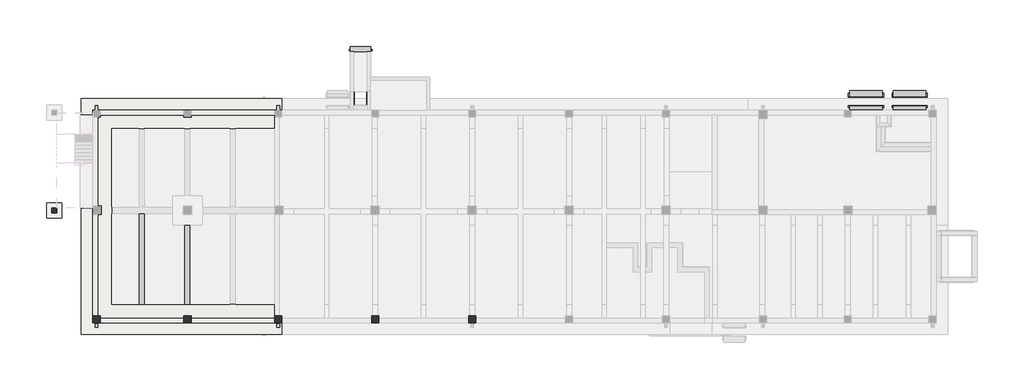
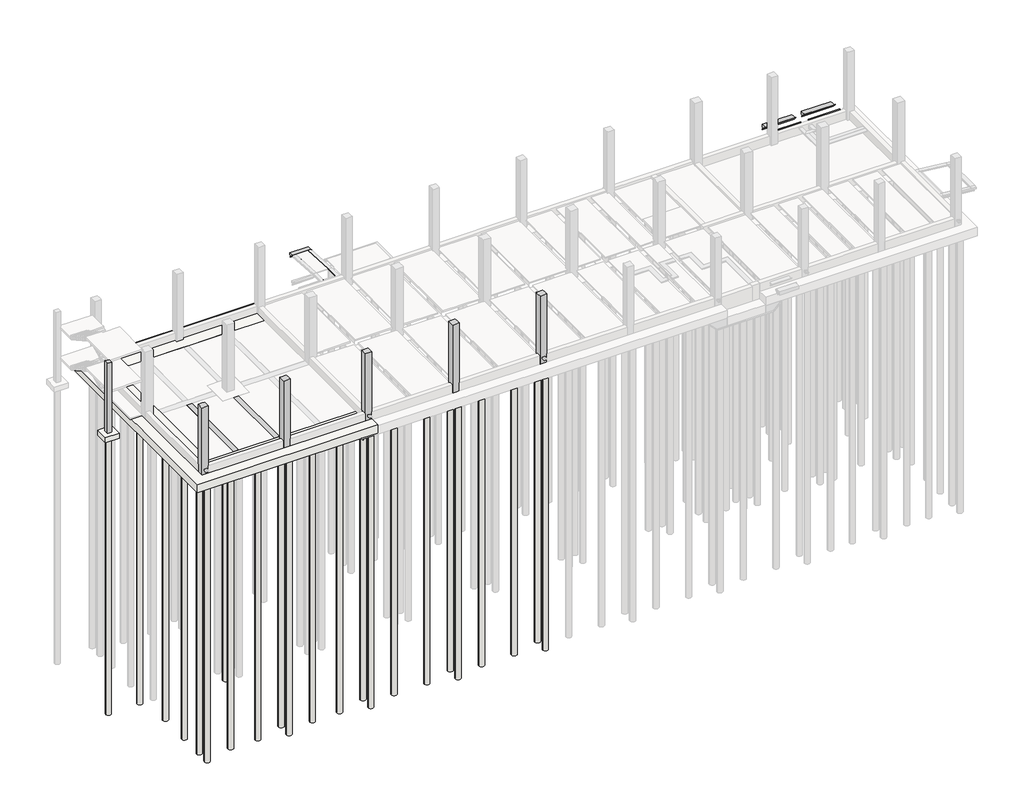
# One storey, part 3 of 7: 26 slabs, 11 proxies, 6 columns, 2 beams.
"""IFC4 building model written with IfcOpenShell, lengths in millimetres."""

from ifc_helpers import new_model, si_unit, point, frame, frame_2d, origin, place, context, project, spatial, polyline, circle_curve, trimmed, segment, composite_curve, outline, extrude, faceted_brep, element, save

model = new_model("IFC4")

# Units and contexts
model_context = context("Model", 3, world=origin())
ifc_project = project(units=[si_unit("LENGTHUNIT", "METRE", prefix="MILLI")], contexts=[model_context])

# Site, building, storey
site = spatial("IfcSite", under=ifc_project)
building = spatial("IfcBuilding", under=site)
storey = spatial("IfcBuildingStorey", under=building, Name="H.P.P", Elevation=4500.0)

# Beams
placement = place(None, origin())
element("IfcBeam", 1, ObjectType="RC Beam_Rectangular : H_SB_AR S16_TG-UG_500x700_FB1A", at=placement, inside=storey, context=model_context, shape_type="Brep", body=[
    faceted_brep([(3500.0, -15750.0, 3400.0), (4000.0, -15750.0, 3400.0), (4000.0, -15750.0, 3840.0), (4000.0, -15750.0, 3950.0), (4000.0, -15750.0, 4100.0), (3500.0, -15750.0, 4100.0), (3500.0, -15750.0, 3950.0), (3500.0, -15750.0, 3840.0), (4000.0, -8300.0, 4100.0), (3500.0, -8300.0, 4100.0), (4000.0, -8300.0, 3950.0), (4000.0, -8300.0, 3400.0), (4000.0, -8300.0, 3840.0), (3500.0, -8300.0, 3400.0), (3500.0, -8300.0, 3950.0), (3500.0, -8300.0, 3840.0)], [[[0, 1, 2, 3, 4, 5, 6, 7]], [[5, 4, 8, 9]], [[10, 8, 4, 3, 2, 1, 11, 12]], [[1, 0, 13, 11]], [[9, 14, 15, 13, 0, 7, 6, 5]], [[9, 8, 10, 12, 11, 13, 15, 14]]]),
])
element("IfcBeam", 2, ObjectType="RC Beam_Rectangular : H_SB_AR S16_TG-UG_500x700_FG1", at=placement, inside=storey, context=model_context, shape_type="Brep", body=[
    faceted_brep([(7250.0, -9250.0, 4100.0), (7750.0, -9250.0, 4100.0), (7750.0, -9250.0, 3950.0), (7750.0, -9250.0, 3840.0), (7750.0, -9250.0, 3400.0), (7250.0, -9250.0, 3400.0), (7250.0, -9250.0, 3840.0), (7250.0, -9250.0, 3950.0), (7250.0, -15750.0, 3400.0), (7750.0, -15750.0, 3400.0), (7750.0, -15750.0, 3840.0), (7750.0, -15750.0, 3950.0), (7750.0, -15750.0, 4100.0), (7250.0, -15750.0, 4100.0), (7250.0, -15750.0, 3950.0), (7250.0, -15750.0, 3840.0)], [[[0, 1, 2, 3, 4, 5, 6, 7]], [[8, 9, 10, 11, 12, 13, 14, 15]], [[1, 0, 13, 12]], [[1, 12, 11, 10, 9, 4, 3, 2]], [[5, 4, 9, 8]], [[13, 0, 7, 6, 5, 8, 15, 14]]]),
])

# Proxies
element("IfcBuildingElementProxy", 3, Name="H_SF_AR_B08_Stoop_T150_FrontEdge", ObjectType="H_SF_AR_B08_Stoop_T150_FrontEdge", at=placement, inside=storey, context=model_context, shape_type="SweptSolid", body=[
    extrude(outline(polyline([(312.0000074, 4450.0), (312.0000074, 4600.0), (662.0000074, 4600.0), (512.0000074, 4450.0), (312.0000074, 4450.0)])), frame((65750.0, 0.0, 0.0), z_axis=(1.0, 0.0, 0.0), x_axis=(0.0, 1.0, 0.0)), (0.0, 0.0, 1.0), 2700.0),
])
element("IfcBuildingElementProxy", 4, Name="H_SF_AR_B08_Stoop_T150_FrontEdge_500x300", ObjectType="H_SF_AR_B08_Stoop_T150_FrontEdge_500x300", at=placement, inside=storey, context=model_context, shape_type="Brep", body=[
    faceted_brep([(68450.0, 1900.0, 4300.0), (68450.0, 1900.0, 4600.0), (68450.0, 1600.0, 4600.0), (68450.0, 1400.0, 4600.0), (68450.0, 1700.0, 4300.0), (65750.0, 1900.0, 4300.0), (65750.0, 1700.0, 4300.0), (65750.0, 1400.0, 4600.0), (65750.0, 1600.0, 4600.0), (65750.0, 1900.0, 4600.0)], [[[0, 1, 2, 3, 4]], [[5, 6, 7, 8, 9]], [[1, 0, 5, 9]], [[3, 2, 1, 9, 8, 7]], [[4, 3, 7, 6]], [[0, 4, 6, 5]]]),
])
element("IfcBuildingElementProxy", 5, Name="H_SF_AR_S18_Lean_T50_300X300", ObjectType="H_SF_AR_S18_Lean_T50_300X300", at=placement, inside=storey, context=model_context, shape_type="SweptSolid", body=[
    extrude(outline(polyline([(1700.0, 4300.0), (1700.0, 4250.0), (1679.2893219, 4250.0), (1379.2893219, 4550.0), (1400.0, 4550.0), (1400.0, 4600.0), (1700.0, 4300.0)])), frame((65650.0, 0.0, 0.0), z_axis=(1.0, 0.0, 0.0), x_axis=(0.0, 1.0, 0.0)), (0.0, 0.0, 1.0), 2900.0),
])
element("IfcBuildingElementProxy", 6, Name="H_SF_AR_S18_Lean_T50_150X150", ObjectType="H_SF_AR_S18_Lean_T50_150X150", at=placement, inside=storey, context=model_context, shape_type="SweptSolid", body=[
    extrude(outline(polyline([(512.0000074, 4400.0), (512.0000074, 4450.0), (662.0000074, 4600.0), (662.0000074, 4550.0), (682.7106855, 4550.0), (532.7106855, 4400.0), (512.0000074, 4400.0)])), frame((65650.0, 0.0, 0.0), z_axis=(1.0, 0.0, 0.0), x_axis=(0.0, 1.0, 0.0)), (0.0, 0.0, 1.0), 2900.0),
])
element("IfcBuildingElementProxy", 7, Name="H_SF_AR_B08_Stoop_T150_FrontEdge", ObjectType="H_SF_AR_B08_Stoop_T150_FrontEdge", at=placement, inside=storey, context=model_context, shape_type="SweptSolid", body=[
    extrude(outline(polyline([(312.0000074, 4450.0), (312.0000074, 4600.0), (662.0000074, 4600.0), (512.0000074, 4450.0), (312.0000074, 4450.0)])), frame((62150.0, 0.0, 0.0), z_axis=(1.0, 0.0, 0.0), x_axis=(0.0, 1.0, 0.0)), (0.0, 0.0, 1.0), 2700.0),
])
element("IfcBuildingElementProxy", 8, Name="H_SF_AR_B08_Stoop_T150_FrontEdge_500x300", ObjectType="H_SF_AR_B08_Stoop_T150_FrontEdge_500x300", at=placement, inside=storey, context=model_context, shape_type="Brep", body=[
    faceted_brep([(64850.0, 1900.0, 4300.0), (64850.0, 1900.0, 4600.0), (64850.0, 1600.0, 4600.0), (64850.0, 1400.0, 4600.0), (64850.0, 1700.0, 4300.0), (62150.0, 1900.0, 4300.0), (62150.0, 1700.0, 4300.0), (62150.0, 1400.0, 4600.0), (62150.0, 1600.0, 4600.0), (62150.0, 1900.0, 4600.0)], [[[0, 1, 2, 3, 4]], [[5, 6, 7, 8, 9]], [[1, 0, 5, 9]], [[3, 2, 1, 9, 8, 7]], [[4, 3, 7, 6]], [[0, 4, 6, 5]]]),
])
element("IfcBuildingElementProxy", 9, Name="H_SF_AR_S18_Lean_T50_300X300", ObjectType="H_SF_AR_S18_Lean_T50_300X300", at=placement, inside=storey, context=model_context, shape_type="SweptSolid", body=[
    extrude(outline(polyline([(1700.0, 4300.0), (1700.0, 4250.0), (1679.2893219, 4250.0), (1379.2893219, 4550.0), (1400.0, 4550.0), (1400.0, 4600.0), (1700.0, 4300.0)])), frame((62050.0, 0.0, 0.0), z_axis=(1.0, 0.0, 0.0), x_axis=(0.0, 1.0, 0.0)), (0.0, 0.0, 1.0), 2900.0),
])
element("IfcBuildingElementProxy", 10, Name="H_SF_AR_S18_Lean_T50_150X150", ObjectType="H_SF_AR_S18_Lean_T50_150X150", at=placement, inside=storey, context=model_context, shape_type="SweptSolid", body=[
    extrude(outline(polyline([(512.0000074, 4400.0), (512.0000074, 4450.0), (662.0000074, 4600.0), (662.0000074, 4550.0), (682.7106855, 4550.0), (532.7106855, 4400.0), (512.0000074, 4400.0)])), frame((62050.0, 0.0, 0.0), z_axis=(1.0, 0.0, 0.0), x_axis=(0.0, 1.0, 0.0)), (0.0, 0.0, 1.0), 2900.0),
])
element("IfcBuildingElementProxy", 11, Name="H_SF_AR_B08_Ramp_T150_FrontEdge(SLOPE)", ObjectType="H_SF_AR_B08_Ramp_T150_FrontEdge(SLOPE)", at=placement, inside=storey, context=model_context, shape_type="Brep", body=[
    faceted_brep([(22638.0, 5300.0, 4179.6670362), (22638.0, 5550.0, 4179.6670362), (22638.0, 5550.0, 4349.6670362), (22638.0, 5100.0, 4379.6670362), (22638.0, 5261.0710326, 4218.5960036), (20938.0, 5550.0, 4179.6670362), (20938.0, 5300.0, 4179.6670362), (20938.0, 5261.0710326, 4218.5960036), (20938.0, 5100.0, 4379.6670362), (20938.0, 5550.0, 4349.6670362), (22338.0, 5100.0, 4379.6670362), (21238.0, 5100.0, 4379.6670362)], [[[0, 1, 2, 3, 4]], [[5, 6, 7, 8, 9]], [[1, 5, 9, 2]], [[1, 0, 6, 5]], [[0, 4, 3, 10, 11, 8, 7, 6]], [[3, 2, 9, 8, 11, 10]]]),
])
element("IfcBuildingElementProxy", 12, Name="H_SF_AR_S18_Lean_T50_200X200", ObjectType="H_SF_AR_S18_Lean_T50_200X200", at=placement, inside=storey, context=model_context, shape_type="Brep", body=[
    faceted_brep([(20838.0, 5300.0, 4179.6670362), (20838.0, 5300.0, 4129.6670362), (20838.0, 5279.2893219, 4129.6670362), (20838.0, 5184.596098, 4224.3602601), (20838.0, 5260.3575388, 4219.3094974), (22738.0, 5300.0, 4129.6670362), (22738.0, 5300.0, 4179.6670362), (22738.0, 5260.3575388, 4219.3094974), (22738.0, 5184.596098, 4224.3602601), (22738.0, 5238.2864422, 4170.6699159), (22738.0, 5279.2893219, 4129.6670362), (20938.0, 5260.3575388, 4219.3094974), (20938.0, 5261.0710326, 4218.5960036), (21088.0, 5261.0710326, 4218.5960036), (21238.0, 5100.0, 4379.6670362), (22338.0, 5100.0, 4379.6670362), (22488.0, 5261.0710326, 4218.5960036), (22638.0, 5261.0710326, 4218.5960036), (22638.0, 5260.3575388, 4219.3094974), (22638.0, 5300.0, 4179.6670362), (20938.0, 5300.0, 4179.6670362), (22638.0, 5184.596098, 4224.3602601), (22638.0, 5185.3095918, 4223.6467663), (22488.0, 5185.3095918, 4223.6467663), (22389.2669117, 5079.2893219, 4329.6670362), (22319.2206862, 5079.2893219, 4329.6670362), (21256.7793138, 5079.2893219, 4329.6670362), (21186.7330883, 5079.2893219, 4329.6670362), (21088.0, 5185.3095918, 4223.6467663), (20938.0, 5185.3095918, 4223.6467663), (20938.0, 5184.596098, 4224.3602601), (20850.0, 5184.596098, 4224.3602601), (22387.8892579, 5100.0, 4329.6670362), (22317.8430324, 5100.0, 4329.6670362), (21258.1569676, 5100.0, 4329.6670362), (21188.1107421, 5100.0, 4329.6670362)], [[[0, 1, 2, 3, 4]], [[5, 6, 7, 8, 9, 10]], [[0, 4, 11, 12, 13, 14, 15, 16, 17, 18, 7, 6, 19, 20]], [[1, 0, 20, 19, 6, 5]], [[2, 1, 5, 10]], [[2, 10, 9, 8, 21, 22, 23, 24, 25, 26, 27, 28, 29, 30, 31, 3]], [[27, 26, 25, 24, 32, 33, 34, 35]], [[15, 14, 35, 34, 33, 32]], [[8, 7, 18, 21]], [[4, 3, 31, 30, 11]], [[29, 12, 11, 30]], [[13, 28, 27, 35, 14]], [[12, 29, 28, 13]], [[17, 22, 21, 18]], [[23, 16, 15, 32, 24]], [[22, 17, 16, 23]]]),
])
element("IfcBuildingElementProxy", 13, Name="H_SF_AR_S18_Lean_T50_150X150", ObjectType="H_SF_AR_S18_Lean_T50_150X150", at=placement, inside=storey, context=model_context, shape_type="Brep", body=[
    faceted_brep([(22338.0, 1800.0, 4600.0), (22488.0, 1800.0, 4450.0), (22488.0, 1800.0, 4400.0), (22467.2893219, 1800.0, 4400.0), (22317.2893219, 1800.0, 4550.0), (22338.0, 1800.0, 4550.0), (22488.0, 550.0, 4450.0), (22338.0, 700.0, 4600.0), (22338.0, 700.0, 4550.0), (22317.2893219, 720.7106781, 4550.0), (22467.2893219, 570.7106781, 4400.0), (22488.0, 550.0, 4400.0)], [[[0, 1, 2, 3, 4, 5]], [[6, 7, 8, 9, 10, 11]], [[1, 0, 7, 6]], [[2, 1, 6, 11]], [[3, 2, 11, 10]], [[4, 3, 10, 9]], [[5, 4, 9, 8]], [[0, 5, 8, 7]]]),
    faceted_brep([(21238.0, 700.0, 4600.0), (21088.0, 550.0, 4450.0), (21088.0, 550.0, 4400.0), (21108.7106781, 570.7106781, 4400.0), (21258.7106781, 720.7106781, 4550.0), (21238.0, 700.0, 4550.0), (21088.0, 1800.0, 4450.0), (21238.0, 1800.0, 4600.0), (21238.0, 1800.0, 4550.0), (21258.7106781, 1800.0, 4550.0), (21108.7106781, 1800.0, 4400.0), (21088.0, 1800.0, 4400.0)], [[[0, 1, 2, 3, 4, 5]], [[6, 7, 8, 9, 10, 11]], [[1, 0, 7, 6]], [[2, 1, 6, 11]], [[3, 2, 11, 10]], [[4, 3, 10, 9]], [[5, 4, 9, 8]], [[0, 5, 8, 7]]]),
    faceted_brep([(22488.0, 1800.0, 4450.0), (22338.0, 1800.0, 4600.3329638), (22338.0, 1800.0, 4550.2219759), (22317.2893219, 1800.0, 4550.2219759), (22467.2893219, 1800.0, 4399.8890121), (22488.0, 1800.0, 4399.8890121), (22488.0, 5184.596098, 4224.3602601), (22389.9313644, 5079.2893219, 4329.6670362), (22388.5537105, 5100.0, 4329.6670362), (22338.6644526, 5100.0, 4379.6670362), (22338.0, 5109.9889135, 4379.6670362), (22488.0, 5238.2864422, 4170.6699159), (22467.2893219, 5238.2864422, 4170.6699159), (22317.2893219, 5100.0, 4330.2219759), (22317.8430324, 5100.0, 4329.6670362), (22319.2206862, 5079.2893219, 4329.6670362), (22338.0, 5100.0, 4330.2219759), (22338.0, 5100.0, 4379.6670362), (22389.2669117, 5079.2893219, 4329.6670362), (22387.8892579, 5100.0, 4329.6670362)], [[[0, 1, 2, 3, 4, 5]], [[1, 0, 6, 7, 8, 9, 10]], [[0, 5, 11, 6]], [[5, 4, 12, 11]], [[4, 3, 13, 14, 15, 12]], [[3, 2, 16, 13]], [[2, 1, 10, 17, 16]], [[10, 9, 17]], [[15, 18, 7, 6, 11, 12]], [[7, 18, 15, 14, 19, 8]], [[8, 19, 14, 13, 16, 17, 9]]]),
    faceted_brep([(21238.0, 1800.0, 4600.3329638), (21088.0, 1800.0, 4450.0), (21088.0, 1800.0, 4399.8890121), (21108.7106781, 1800.0, 4399.8890121), (21258.7106781, 1800.0, 4550.2219759), (21238.0, 1800.0, 4550.2219759), (21238.0, 5109.9889135, 4379.6670362), (21237.3355474, 5100.0, 4379.6670362), (21187.4462895, 5100.0, 4329.6670362), (21186.0686356, 5079.2893219, 4329.6670362), (21088.0, 5184.596098, 4224.3602601), (21088.0, 5238.2864422, 4170.6699159), (21108.7106781, 5238.2864422, 4170.6699159), (21256.7793138, 5079.2893219, 4329.6670362), (21258.1569676, 5100.0, 4329.6670362), (21258.7106781, 5100.0, 4330.2219759), (21238.0, 5100.0, 4330.2219759), (21238.0, 5100.0, 4379.6670362), (21186.7330883, 5079.2893219, 4329.6670362), (21188.1107421, 5100.0, 4329.6670362)], [[[0, 1, 2, 3, 4, 5]], [[1, 0, 6, 7, 8, 9, 10]], [[2, 1, 10, 11]], [[3, 2, 11, 12]], [[4, 3, 12, 13, 14, 15]], [[5, 4, 15, 16]], [[0, 5, 16, 17, 6]], [[7, 6, 17]], [[9, 18, 13, 12, 11, 10]], [[13, 18, 9, 8, 19, 14]], [[14, 19, 8, 7, 17, 16, 15]]]),
])

# Columns
element("IfcColumn", 14, ObjectType="RC_Column_Rectangular : H_SC_AR S15_RC Col-AG_600x600_C2", at=placement, inside=storey, context=model_context, shape_type="Brep", body=[
    faceted_brep([(30700.0, -16700.0, 4000.0), (31300.0, -16700.0, 4000.0), (31300.0, -16900.0, 4000.0), (31300.0, -17300.0, 4000.0), (30700.0, -17300.0, 4000.0), (30700.0, -16900.0, 4000.0), (30700.0, -16700.0, 4650.0), (30700.0, -16700.0, 4800.0), (30700.0, -16700.0, 10450.0), (30700.0, -16700.0, 10600.0), (30750.0000002, -16700.0, 10600.0), (31249.9999998, -16700.0, 10600.0), (31300.0, -16700.0, 10600.0), (31300.0, -16700.0, 10450.0), (31300.0, -16700.0, 4800.0), (31300.0, -16700.0, 4650.0), (31300.0, -16900.0, 10600.0), (31300.0, -17300.0, 10600.0), (31300.0, -17300.0, 9800.0), (31300.0, -17300.0, 4800.0), (30700.0, -17300.0, 10600.0), (30700.0, -17300.0, 9800.0), (30700.0, -17300.0, 4800.0), (30700.0, -16900.0, 10600.0)], [[[0, 1, 2, 3, 4, 5]], [[1, 0, 6, 7, 8, 9, 10, 11, 12, 13, 14, 15]], [[3, 2, 1, 15, 14, 13, 12, 16, 17, 18, 19]], [[4, 3, 19, 18, 17, 20, 21, 22]], [[0, 5, 4, 22, 21, 20, 23, 9, 8, 7, 6]], [[20, 17, 16, 12, 11, 10, 9, 23]]]),
])
element("IfcColumn", 15, ObjectType="RC_Column_Rectangular : H_SC_AR S15_RC Col-AG_600x600_C2", at=placement, inside=storey, context=model_context, shape_type="Brep", body=[
    faceted_brep([(22700.0, -16700.0, 4000.0), (23300.0, -16700.0, 4000.0), (23300.0, -16900.0, 4000.0), (23300.0, -17300.0, 4000.0), (22700.0, -17300.0, 4000.0), (22700.0, -16900.0, 4000.0), (22700.0, -16700.0, 4650.0), (22700.0, -16700.0, 4800.0), (22700.0, -16700.0, 10450.0), (22700.0, -16700.0, 10600.0), (23200.0, -16700.0, 10600.0), (23300.0, -16700.0, 10600.0), (23300.0, -16700.0, 10450.0), (23300.0, -16700.0, 4800.0), (23300.0, -16700.0, 4650.0), (23300.0, -16900.0, 10600.0), (23300.0, -17300.0, 10600.0), (23300.0, -17300.0, 9800.0), (23300.0, -17300.0, 4800.0), (22700.0, -17300.0, 10600.0), (22700.0, -17300.0, 9800.0), (22700.0, -17300.0, 4800.0), (22700.0, -16900.0, 10600.0)], [[[0, 1, 2, 3, 4, 5]], [[1, 0, 6, 7, 8, 9, 10, 11, 12, 13, 14]], [[3, 2, 1, 14, 13, 12, 11, 15, 16, 17, 18]], [[4, 3, 18, 17, 16, 19, 20, 21]], [[0, 5, 4, 21, 20, 19, 22, 9, 8, 7, 6]], [[19, 16, 15, 11, 10, 9, 22]]]),
])
element("IfcColumn", 16, ObjectType="RC_Column_Rectangular : H_SC_AR S15_RC Col-AG_600x600_C2", at=placement, inside=storey, context=model_context, shape_type="Brep", body=[
    faceted_brep([(14700.0, -16700.0, 4100.0), (15100.0, -16700.0, 4100.0), (15300.0, -16700.0, 4100.0), (15300.0, -17300.0, 4100.0), (14700.0, -17300.0, 4100.0), (14700.0, -16900.0, 4100.0), (14700.0, -16700.0, 4800.0), (14700.0, -16700.0, 10450.0), (14700.0, -16700.0, 10600.0), (15200.0, -16700.0, 10600.0), (15300.0, -16700.0, 10600.0), (15300.0, -16700.0, 10450.0), (15300.0, -16700.0, 4800.0), (15300.0, -16700.0, 4650.0), (15300.0, -16900.0, 10600.0), (15300.0, -17300.0, 10600.0), (15300.0, -17300.0, 9800.0), (15300.0, -17300.0, 4800.0), (14700.0, -17300.0, 10600.0), (14700.0, -17300.0, 9800.0), (14700.0, -17300.0, 4800.0), (14700.0, -16900.0, 10600.0)], [[[0, 1, 2, 3, 4, 5]], [[2, 1, 0, 6, 7, 8, 9, 10, 11, 12, 13]], [[3, 2, 13, 12, 11, 10, 14, 15, 16, 17]], [[4, 3, 17, 16, 15, 18, 19, 20]], [[0, 5, 4, 20, 19, 18, 21, 8, 7, 6]], [[18, 15, 14, 10, 9, 8, 21]]]),
])
element("IfcColumn", 17, ObjectType="RC_Column_Rectangular : H_SC_AR S15_RC Col-AG_600x600_C2", at=placement, inside=storey, context=model_context, shape_type="Brep", body=[
    faceted_brep([(7200.0, -16700.0, 4100.0), (7800.0, -16700.0, 4100.0), (7800.0, -16900.0, 4100.0), (7800.0, -17300.0, 4100.0), (7200.0, -17300.0, 4100.0), (7200.0, -16900.0, 4100.0), (7200.0, -16700.0, 10450.0), (7200.0, -16700.0, 10600.0), (7250.0, -16700.0, 10600.0), (7750.0, -16700.0, 10600.0), (7800.0, -16700.0, 10600.0), (7800.0, -16700.0, 10450.0), (7800.0, -16900.0, 10600.0), (7800.0, -17300.0, 10600.0), (7800.0, -17300.0, 9800.0), (7800.0, -17300.0, 4800.0), (7200.0, -17300.0, 10600.0), (7200.0, -17300.0, 9800.0), (7200.0, -17300.0, 4800.0), (7200.0, -16900.0, 10600.0)], [[[0, 1, 2, 3, 4, 5]], [[1, 0, 6, 7, 8, 9, 10, 11]], [[3, 2, 1, 11, 10, 12, 13, 14, 15]], [[4, 3, 15, 14, 13, 16, 17, 18]], [[0, 5, 4, 18, 17, 16, 19, 7, 6]], [[16, 13, 12, 10, 9, 8, 7, 19]]]),
])
element("IfcColumn", 18, ObjectType="RC_Column_Rectangular : H_SC_AR S15_RC Col-AG_600x600_C2", at=placement, inside=storey, context=model_context, shape_type="Brep", body=[
    faceted_brep([(-300.0, -16700.0, 4100.0), (100.0, -16700.0, 4100.0), (300.0, -16700.0, 4100.0), (300.0, -16900.0, 4100.0), (300.0, -17300.0, 4100.0), (-300.0, -17300.0, 4100.0), (-300.0, -16700.0, 4800.0), (-300.0, -16700.0, 9900.0), (-300.0, -16700.0, 10600.0), (100.0, -16700.0, 10600.0), (300.0, -16700.0, 10600.0), (300.0, -16700.0, 10450.0), (300.0, -16900.0, 10600.0), (300.0, -17300.0, 10600.0), (300.0, -17300.0, 9800.0), (300.0, -17300.0, 4800.0), (-300.0, -17300.0, 10600.0)], [[[0, 1, 2, 3, 4, 5]], [[2, 1, 0, 6, 7, 8, 9, 10, 11]], [[4, 3, 2, 11, 10, 12, 13, 14, 15]], [[5, 4, 15, 14, 13, 16]], [[0, 5, 16, 8, 7, 6]], [[16, 13, 12, 10, 9, 8]]]),
])
element("IfcColumn", 19, ObjectType="RC_Column_Rectangular : H_SC_AR S15_RC Col-AG_400x400_C3", at=placement, inside=storey, context=model_context, shape_type="Brep", body=[
    faceted_brep([(-3300.0, -7800.0, 3800.0), (-3300.0, -8200.0, 3800.0), (-3700.0, -8200.0, 3800.0), (-3700.0, -7800.0, 3800.0), (-3300.0, -7800.0, 10600.0), (-3300.0, -8200.0, 10600.0), (-3300.0, -7800.0, 4030.0), (-3300.0, -7800.0, 4630.0), (-3300.0, -7800.0, 6990.0), (-3300.0, -7800.0, 7590.0), (-3300.0, -7800.0, 9950.0), (-3300.0, -7800.0, 10550.0), (-3700.0, -8200.0, 10600.0), (-3700.0, -7800.0, 10600.0), (-3700.0, -7800.0, 10550.0), (-3700.0, -7800.0, 9950.0), (-3700.0, -7800.0, 7590.0), (-3700.0, -7800.0, 6990.0), (-3700.0, -7800.0, 4630.0), (-3700.0, -7800.0, 4030.0)], [[[0, 1, 2, 3]], [[4, 5, 1, 0, 6, 7, 8, 9, 10, 11]], [[5, 12, 2, 1]], [[12, 13, 14, 15, 16, 17, 18, 19, 3, 2]], [[13, 4, 11, 10, 9, 8, 7, 6, 0, 3, 19, 18, 17, 16, 15, 14]], [[4, 13, 12, 5]]]),
])

# Slabs
element("IfcSlab", 20, ObjectType="H_SF_AR S18_MAT_T800_WF1", at=placement, inside=storey, context=model_context, shape_type="Brep", body=[
    faceted_brep([(15299.9999999, 1249.9999999, 3300.0), (15299.9999999, -1250.0000001, 3300.0), (13799.9999999, -1250.0000001, 3300.0), (1250.0000002, -1250.0000001, 3300.0), (1250.0000002, -7700.0, 3300.0), (1250.0000002, -8300.0, 3300.0), (1250.0000002, -15750.0000001, 3300.0), (13799.9999999, -15750.0000001, 3300.0), (15299.9999999, -15750.0000001, 3300.0), (15299.9999999, -18250.0000001, 3300.0), (13799.9999999, -18250.0000001, 3300.0), (-1250.0, -18250.0000001, 3300.0), (-1250.0, 1249.9999999, 3300.0), (13799.9999999, 1249.9999999, 3300.0), (15299.9999999, 1249.9999999, 4100.0), (-1250.0, 1249.9999999, 4100.0), (-1250.0, -18250.0000001, 4100.0), (15299.9999999, -18250.0000001, 4100.0), (15299.9999999, -15750.0000001, 4100.0), (15200.0, -15750.0000001, 4100.0), (14700.0, -15750.0000001, 4100.0), (11500.0, -15750.0000001, 4100.0), (11000.0, -15750.0000001, 4100.0), (7750.0, -15750.0000001, 4100.0), (7250.0, -15750.0000001, 4100.0), (4000.0, -15750.0000001, 4100.0), (3500.0, -15750.0000001, 4100.0), (1250.0000002, -15750.0000001, 4100.0), (1250.0000002, -8300.0, 4100.0), (1250.0000002, -7700.0, 4100.0), (1250.0000002, -1250.0000001, 4100.0), (3500.0, -1250.0000001, 4100.0), (4000.0, -1250.0000001, 4100.0), (7250.0, -1250.0000001, 4100.0), (7750.0, -1250.0000001, 4100.0), (11000.0, -1250.0000001, 4100.0), (11500.0, -1250.0000001, 4100.0), (14700.0, -1250.0000001, 4100.0), (15200.0, -1250.0000001, 4100.0), (15299.9999999, -1250.0000001, 4100.0), (15299.9999999, -18250.0000001, 4000.0), (15299.9999999, 1249.9999999, 4000.0), (15299.9999999, -15750.0000001, 4000.0), (15299.9999999, -1250.0000001, 4000.0)], [[[0, 1, 2, 3, 4, 5, 6, 7, 8, 9, 10, 11, 12, 13]], [[14, 15, 16, 17, 18, 19, 20, 21, 22, 23, 24, 25, 26, 27, 28, 29, 30, 31, 32, 33, 34, 35, 36, 37, 38, 39]], [[11, 10, 9, 40, 17, 16]], [[12, 11, 16, 15]], [[0, 13, 12, 15, 14, 41]], [[6, 5, 4, 3, 30, 29, 28, 27]], [[8, 7, 6, 27, 26, 25, 24, 23, 22, 21, 20, 19, 18, 42]], [[3, 2, 1, 43, 39, 38, 37, 36, 35, 34, 33, 32, 31, 30]], [[1, 0, 41, 14, 39, 43]], [[9, 8, 42, 18, 17, 40]]]),
])
element("IfcSlab", 21, ObjectType="H_SF_AR_S18_Lean_T50", at=placement, inside=storey, context=model_context, shape_type="SweptSolid", body=[
    extrude(outline(polyline([(3390.0, -1360.0000001), (3390.0, -7590.0), (1360.0000002, -7590.0), (1360.0000002, -1360.0000001), (3390.0, -1360.0000001)])), frame((0.0, 0.0, 3790.0), z_axis=(0.0, 0.0, 1.0), x_axis=(1.0, 0.0, 0.0)), (0.0, 0.0, 1.0), 50.0),
    extrude(outline(polyline([(3390.0, -8410.0), (3390.0, -15640.0000001), (1360.0000002, -15640.0000001), (1360.0000002, -8410.0), (3390.0, -8410.0)])), frame((0.0, 0.0, 3790.0), z_axis=(0.0, 0.0, 1.0), x_axis=(1.0, 0.0, 0.0)), (0.0, 0.0, 1.0), 50.0),
    extrude(outline(polyline([(6250.0, -8410.0), (6250.0, -9250.0), (7140.0, -9250.0), (7140.0, -15640.0000001), (4110.0, -15640.0000001), (4110.0, -8410.0), (6250.0, -8410.0)])), frame((0.0, 0.0, 3790.0), z_axis=(0.0, 0.0, 1.0), x_axis=(1.0, 0.0, 0.0)), (0.0, 0.0, 1.0), 50.0),
    extrude(outline(polyline([(6250.0, -7590.0), (4110.0, -7590.0), (4110.0, -1360.0000001), (7140.0, -1360.0000001), (7140.0, -6750.0), (6250.0, -6750.0), (6250.0, -7590.0)])), frame((0.0, 0.0, 3790.0), z_axis=(0.0, 0.0, 1.0), x_axis=(1.0, 0.0, 0.0)), (0.0, 0.0, 1.0), 50.0),
    extrude(outline(polyline([(8750.0, -8410.0), (10890.0, -8410.0), (10890.0, -15640.0000001), (7860.0, -15640.0000001), (7860.0, -9250.0), (8750.0, -9250.0), (8750.0, -8410.0)])), frame((0.0, 0.0, 3790.0), z_axis=(0.0, 0.0, 1.0), x_axis=(1.0, 0.0, 0.0)), (0.0, 0.0, 1.0), 50.0),
    extrude(outline(polyline([(8750.0, -7590.0), (8750.0, -6750.0), (7860.0, -6750.0), (7860.0, -1360.0000001), (10890.0, -1360.0000001), (10890.0, -7590.0), (8750.0, -7590.0)])), frame((0.0, 0.0, 3790.0), z_axis=(0.0, 0.0, 1.0), x_axis=(1.0, 0.0, 0.0)), (0.0, 0.0, 1.0), 50.0),
    extrude(outline(polyline([(13800.0000001, -8410.0), (13800.0000001, -9250.0), (14590.0, -9250.0), (14590.0, -15640.0000001), (11610.0, -15640.0000001), (11610.0, -8410.0), (13800.0000001, -8410.0)])), frame((0.0, 0.0, 3790.0), z_axis=(0.0, 0.0, 1.0), x_axis=(1.0, 0.0, 0.0)), (0.0, 0.0, 1.0), 50.0),
    extrude(outline(polyline([(13800.0000001, -7590.0), (11610.0, -7590.0), (11610.0, -1360.0000001), (14590.0, -1360.0000001), (14590.0, -6750.0), (13800.0000001, -6750.0), (13800.0000001, -7590.0)])), frame((0.0, 0.0, 3790.0), z_axis=(0.0, 0.0, 1.0), x_axis=(1.0, 0.0, 0.0)), (0.0, 0.0, 1.0), 50.0),
])
element("IfcSlab", 22, ObjectType="Foundation Rectangular (Non-Pile) : H_SF_AR S18_Ret Fdn_1250x1250xT500_F2", at=placement, inside=storey, context=model_context, shape_type="SweptSolid", body=[
    extrude(outline(polyline([(-2875.0, -7375.0), (-2875.0, -8625.0), (-4125.0, -8625.0), (-4125.0, -7375.0), (-2875.0, -7375.0)])), frame((0.0, 0.0, 3300.0), z_axis=(0.0, 0.0, 1.0), x_axis=(1.0, 0.0, 0.0)), (0.0, 0.0, 1.0), 500.0),
])
element("IfcSlab", 23, ObjectType="PILE : H_FL_AR S19_Pile_D500_L26.9", at=placement, inside=storey, context=model_context, shape_type="SweptSolid", body=[
    extrude(outline(composite_curve([segment(trimmed(circle_curve(frame_2d((-3500.0, -8000.0)), 250.0), [point((-3750.0, -8000.0))], [point((-3250.0, -8000.0))], False, "CARTESIAN"), True, "CONTINUOUS"), segment(trimmed(circle_curve(frame_2d((-3500.0, -8000.0)), 250.0), [point((-3250.0, -8000.0))], [point((-3750.0, -8000.0))], False, "CARTESIAN"), True, "CONTINUOUS")], self_intersect=False)), frame((0.0, 0.0, -23500.0), z_axis=(0.0, 0.0, 1.0), x_axis=(1.0, 0.0, 0.0)), (0.0, 0.0, 1.0), 26750.0),
])
element("IfcSlab", 24, ObjectType="PILE : H_FL_AR S19_Pile_D500_L26.9", at=placement, inside=storey, context=model_context, shape_type="SweptSolid", body=[
    extrude(outline(composite_curve([segment(trimmed(circle_curve(frame_2d((-625.0000004, -8000.0)), 250.0), [point((-875.0000004, -8000.0))], [point((-375.0000004, -8000.0))], False, "CARTESIAN"), True, "CONTINUOUS"), segment(trimmed(circle_curve(frame_2d((-625.0000004, -8000.0)), 250.0), [point((-375.0000004, -8000.0))], [point((-875.0000004, -8000.0))], False, "CARTESIAN"), True, "CONTINUOUS")], self_intersect=False)), frame((0.0, 0.0, -23500.0), z_axis=(0.0, 0.0, 1.0), x_axis=(1.0, 0.0, 0.0)), (0.0, 0.0, 1.0), 26750.0),
])
element("IfcSlab", 25, ObjectType="PILE : H_FL_AR S19_Pile_D500_L26.9", at=placement, inside=storey, context=model_context, shape_type="SweptSolid", body=[
    extrude(outline(composite_curve([segment(trimmed(circle_curve(frame_2d((0.0, -11000.0000003)), 250.0), [point((-250.0, -11000.0000003))], [point((250.0, -11000.0000003))], False, "CARTESIAN"), True, "CONTINUOUS"), segment(trimmed(circle_curve(frame_2d((0.0, -11000.0000003)), 250.0), [point((250.0, -11000.0000003))], [point((-250.0, -11000.0000003))], False, "CARTESIAN"), True, "CONTINUOUS")], self_intersect=False)), frame((0.0, 0.0, -23500.0), z_axis=(0.0, 0.0, 1.0), x_axis=(1.0, 0.0, 0.0)), (0.0, 0.0, 1.0), 26750.0),
])
element("IfcSlab", 26, ObjectType="PILE : H_FL_AR S19_Pile_D500_L26.9", at=placement, inside=storey, context=model_context, shape_type="SweptSolid", body=[
    extrude(outline(composite_curve([segment(trimmed(circle_curve(frame_2d((0.0, -14000.0000004)), 250.0), [point((-250.0, -14000.0000004))], [point((250.0, -14000.0000004))], False, "CARTESIAN"), True, "CONTINUOUS"), segment(trimmed(circle_curve(frame_2d((0.0, -14000.0000004)), 250.0), [point((250.0, -14000.0000004))], [point((-250.0, -14000.0000004))], False, "CARTESIAN"), True, "CONTINUOUS")], self_intersect=False)), frame((0.0, 0.0, -23500.0), z_axis=(0.0, 0.0, 1.0), x_axis=(1.0, 0.0, 0.0)), (0.0, 0.0, 1.0), 26750.0),
])
element("IfcSlab", 27, ObjectType="PILE : H_FL_AR S19_Pile_D500_L26.7", at=placement, inside=storey, context=model_context, shape_type="SweptSolid", body=[
    extrude(outline(composite_curve([segment(trimmed(circle_curve(frame_2d((6875.0000004, -8624.9999999)), 250.0), [point((6625.0000004, -8624.9999999))], [point((7125.0000004, -8624.9999999))], False, "CARTESIAN"), True, "CONTINUOUS"), segment(trimmed(circle_curve(frame_2d((6875.0000004, -8624.9999999)), 250.0), [point((7125.0000004, -8624.9999999))], [point((6625.0000004, -8624.9999999))], False, "CARTESIAN"), True, "CONTINUOUS")], self_intersect=False)), frame((0.0, 0.0, -23500.0), z_axis=(0.0, 0.0, 1.0), x_axis=(1.0, 0.0, 0.0)), (0.0, 0.0, 1.0), 26550.0),
])
element("IfcSlab", 28, ObjectType="PILE : H_FL_AR S19_Pile_D500_L26.9", at=placement, inside=storey, context=model_context, shape_type="SweptSolid", body=[
    extrude(outline(composite_curve([segment(trimmed(circle_curve(frame_2d((0.0, -16375.0000004)), 250.0), [point((-250.0, -16375.0000004))], [point((250.0, -16375.0000004))], False, "CARTESIAN"), True, "CONTINUOUS"), segment(trimmed(circle_curve(frame_2d((0.0, -16375.0000004)), 250.0), [point((250.0, -16375.0000004))], [point((-250.0, -16375.0000004))], False, "CARTESIAN"), True, "CONTINUOUS")], self_intersect=False)), frame((0.0, 0.0, -23500.0), z_axis=(0.0, 0.0, 1.0), x_axis=(1.0, 0.0, 0.0)), (0.0, 0.0, 1.0), 26750.0),
])
element("IfcSlab", 29, ObjectType="PILE : H_FL_AR S19_Pile_D500_L26.9", at=placement, inside=storey, context=model_context, shape_type="SweptSolid", body=[
    extrude(outline(composite_curve([segment(trimmed(circle_curve(frame_2d((0.0, -17625.0)), 250.0), [point((-250.0, -17625.0))], [point((250.0, -17625.0))], False, "CARTESIAN"), True, "CONTINUOUS"), segment(trimmed(circle_curve(frame_2d((0.0, -17625.0)), 250.0), [point((250.0, -17625.0))], [point((-250.0, -17625.0))], False, "CARTESIAN"), True, "CONTINUOUS")], self_intersect=False)), frame((0.0, 0.0, -23500.0), z_axis=(0.0, 0.0, 1.0), x_axis=(1.0, 0.0, 0.0)), (0.0, 0.0, 1.0), 26750.0),
])
element("IfcSlab", 30, ObjectType="PILE : H_FL_AR S19_Pile_D500_L26.9", at=placement, inside=storey, context=model_context, shape_type="SweptSolid", body=[
    extrude(outline(composite_curve([segment(trimmed(circle_curve(frame_2d((2506.7380833, -17000.0)), 250.0), [point((2256.7380833, -17000.0))], [point((2756.7380833, -17000.0))], False, "CARTESIAN"), True, "CONTINUOUS"), segment(trimmed(circle_curve(frame_2d((2506.7380833, -17000.0)), 250.0), [point((2756.7380833, -17000.0))], [point((2256.7380833, -17000.0))], False, "CARTESIAN"), True, "CONTINUOUS")], self_intersect=False)), frame((0.0, 0.0, -23500.0), z_axis=(0.0, 0.0, 1.0), x_axis=(1.0, 0.0, 0.0)), (0.0, 0.0, 1.0), 26750.0),
])
element("IfcSlab", 31, ObjectType="PILE : H_FL_AR S19_Pile_D500_L26.9", at=placement, inside=storey, context=model_context, shape_type="SweptSolid", body=[
    extrude(outline(composite_curve([segment(trimmed(circle_curve(frame_2d((5000.0000002, -17000.0)), 250.0), [point((4750.0000002, -17000.0))], [point((5250.0000002, -17000.0))], False, "CARTESIAN"), True, "CONTINUOUS"), segment(trimmed(circle_curve(frame_2d((5000.0000002, -17000.0)), 250.0), [point((5250.0000002, -17000.0))], [point((4750.0000002, -17000.0))], False, "CARTESIAN"), True, "CONTINUOUS")], self_intersect=False)), frame((0.0, 0.0, -23500.0), z_axis=(0.0, 0.0, 1.0), x_axis=(1.0, 0.0, 0.0)), (0.0, 0.0, 1.0), 26750.0),
])
element("IfcSlab", 32, ObjectType="PILE : H_FL_AR S19_Pile_D500_L26.9", at=placement, inside=storey, context=model_context, shape_type="SweptSolid", body=[
    extrude(outline(composite_curve([segment(trimmed(circle_curve(frame_2d((7500.0, -16375.0000002)), 250.0), [point((7250.0, -16375.0000002))], [point((7750.0, -16375.0000002))], False, "CARTESIAN"), True, "CONTINUOUS"), segment(trimmed(circle_curve(frame_2d((7500.0, -16375.0000002)), 250.0), [point((7750.0, -16375.0000002))], [point((7250.0, -16375.0000002))], False, "CARTESIAN"), True, "CONTINUOUS")], self_intersect=False)), frame((0.0, 0.0, -23500.0), z_axis=(0.0, 0.0, 1.0), x_axis=(1.0, 0.0, 0.0)), (0.0, 0.0, 1.0), 26750.0),
])
element("IfcSlab", 33, ObjectType="PILE : H_FL_AR S19_Pile_D500_L26.9", at=placement, inside=storey, context=model_context, shape_type="SweptSolid", body=[
    extrude(outline(composite_curve([segment(trimmed(circle_curve(frame_2d((7500.0, -17624.9999998)), 250.0), [point((7250.0, -17624.9999998))], [point((7750.0, -17624.9999998))], False, "CARTESIAN"), True, "CONTINUOUS"), segment(trimmed(circle_curve(frame_2d((7500.0, -17624.9999998)), 250.0), [point((7750.0, -17624.9999998))], [point((7250.0, -17624.9999998))], False, "CARTESIAN"), True, "CONTINUOUS")], self_intersect=False)), frame((0.0, 0.0, -23500.0), z_axis=(0.0, 0.0, 1.0), x_axis=(1.0, 0.0, 0.0)), (0.0, 0.0, 1.0), 26750.0),
])
element("IfcSlab", 34, ObjectType="PILE : H_FL_AR S19_Pile_D500_L26.9", at=placement, inside=storey, context=model_context, shape_type="SweptSolid", body=[
    extrude(outline(composite_curve([segment(trimmed(circle_curve(frame_2d((10000.0000006, -17000.0)), 250.0), [point((9750.0000006, -17000.0))], [point((10250.0000006, -17000.0))], False, "CARTESIAN"), True, "CONTINUOUS"), segment(trimmed(circle_curve(frame_2d((10000.0000006, -17000.0)), 250.0), [point((10250.0000006, -17000.0))], [point((9750.0000006, -17000.0))], False, "CARTESIAN"), True, "CONTINUOUS")], self_intersect=False)), frame((0.0, 0.0, -23500.0), z_axis=(0.0, 0.0, 1.0), x_axis=(1.0, 0.0, 0.0)), (0.0, 0.0, 1.0), 26750.0),
])
element("IfcSlab", 35, ObjectType="PILE : H_FL_AR S19_Pile_D500_L26.9", at=placement, inside=storey, context=model_context, shape_type="SweptSolid", body=[
    extrude(outline(composite_curve([segment(trimmed(circle_curve(frame_2d((12500.0000009, -17000.0)), 250.0), [point((12250.0000009, -17000.0))], [point((12750.0000009, -17000.0))], False, "CARTESIAN"), True, "CONTINUOUS"), segment(trimmed(circle_curve(frame_2d((12500.0000009, -17000.0)), 250.0), [point((12750.0000009, -17000.0))], [point((12250.0000009, -17000.0))], False, "CARTESIAN"), True, "CONTINUOUS")], self_intersect=False)), frame((0.0, 0.0, -23500.0), z_axis=(0.0, 0.0, 1.0), x_axis=(1.0, 0.0, 0.0)), (0.0, 0.0, 1.0), 26750.0),
])
element("IfcSlab", 36, ObjectType="PILE : H_FL_AR S19_Pile_D500_L26.8", at=placement, inside=storey, context=model_context, shape_type="SweptSolid", body=[
    extrude(outline(composite_curve([segment(trimmed(circle_curve(frame_2d((14999.9999999, -16375.0000004)), 250.0), [point((15249.9999999, -16375.0000004))], [point((14749.9999999, -16375.0000004))], False, "CARTESIAN"), True, "CONTINUOUS"), segment(trimmed(circle_curve(frame_2d((14999.9999999, -16375.0000004)), 250.0), [point((14749.9999999, -16375.0000004))], [point((15249.9999999, -16375.0000004))], False, "CARTESIAN"), True, "CONTINUOUS")], self_intersect=False)), frame((0.0, 0.0, 3200.0), z_axis=(0.0, 0.0, 1.0), x_axis=(1.0, 0.0, 0.0)), (0.0, 0.0, 1.0), 100.0),
    extrude(outline(composite_curve([segment(trimmed(circle_curve(frame_2d((14999.9999999, -16375.0000004)), 250.0), [point((14749.9999999, -16375.0000004))], [point((15249.9999999, -16375.0000004))], False, "CARTESIAN"), True, "CONTINUOUS"), segment(trimmed(circle_curve(frame_2d((14999.9999999, -16375.0000004)), 250.0), [point((15249.9999999, -16375.0000004))], [point((14749.9999999, -16375.0000004))], False, "CARTESIAN"), True, "CONTINUOUS")], self_intersect=False)), frame((0.0, 0.0, -23500.0), z_axis=(0.0, 0.0, 1.0), x_axis=(1.0, 0.0, 0.0)), (0.0, 0.0, 1.0), 26650.0),
])
element("IfcSlab", 37, ObjectType="PILE : H_FL_AR S19_Pile_D500_L26.8", at=placement, inside=storey, context=model_context, shape_type="SweptSolid", body=[
    extrude(outline(composite_curve([segment(trimmed(circle_curve(frame_2d((14999.9999999, -17625.0)), 250.0), [point((15249.9999999, -17625.0))], [point((14749.9999999, -17625.0))], False, "CARTESIAN"), True, "CONTINUOUS"), segment(trimmed(circle_curve(frame_2d((14999.9999999, -17625.0)), 250.0), [point((14749.9999999, -17625.0))], [point((15249.9999999, -17625.0))], False, "CARTESIAN"), True, "CONTINUOUS")], self_intersect=False)), frame((0.0, 0.0, 3200.0), z_axis=(0.0, 0.0, 1.0), x_axis=(1.0, 0.0, 0.0)), (0.0, 0.0, 1.0), 100.0),
    extrude(outline(composite_curve([segment(trimmed(circle_curve(frame_2d((14999.9999999, -17625.0)), 250.0), [point((14749.9999999, -17625.0))], [point((15249.9999999, -17625.0))], False, "CARTESIAN"), True, "CONTINUOUS"), segment(trimmed(circle_curve(frame_2d((14999.9999999, -17625.0)), 250.0), [point((15249.9999999, -17625.0))], [point((14749.9999999, -17625.0))], False, "CARTESIAN"), True, "CONTINUOUS")], self_intersect=False)), frame((0.0, 0.0, -23500.0), z_axis=(0.0, 0.0, 1.0), x_axis=(1.0, 0.0, 0.0)), (0.0, 0.0, 1.0), 26650.0),
])
element("IfcSlab", 38, ObjectType="PILE : H_FL_AR S19_Pile_D500_L26.8", at=placement, inside=storey, context=model_context, shape_type="SweptSolid", body=[
    extrude(outline(composite_curve([segment(trimmed(circle_curve(frame_2d((17500.0000012, -17000.0)), 250.0), [point((17250.0000012, -17000.0))], [point((17750.0000012, -17000.0))], False, "CARTESIAN"), True, "CONTINUOUS"), segment(trimmed(circle_curve(frame_2d((17500.0000012, -17000.0)), 250.0), [point((17750.0000012, -17000.0))], [point((17250.0000012, -17000.0))], False, "CARTESIAN"), True, "CONTINUOUS")], self_intersect=False)), frame((0.0, 0.0, -23500.0), z_axis=(0.0, 0.0, 1.0), x_axis=(1.0, 0.0, 0.0)), (0.0, 0.0, 1.0), 26650.0),
])
element("IfcSlab", 39, ObjectType="PILE : H_FL_AR S19_Pile_D500_L26.8", at=placement, inside=storey, context=model_context, shape_type="SweptSolid", body=[
    extrude(outline(composite_curve([segment(trimmed(circle_curve(frame_2d((20500.0000002, -17000.0)), 250.0), [point((20250.0000002, -17000.0))], [point((20750.0000002, -17000.0))], False, "CARTESIAN"), True, "CONTINUOUS"), segment(trimmed(circle_curve(frame_2d((20500.0000002, -17000.0)), 250.0), [point((20750.0000002, -17000.0))], [point((20250.0000002, -17000.0))], False, "CARTESIAN"), True, "CONTINUOUS")], self_intersect=False)), frame((0.0, 0.0, -23500.0), z_axis=(0.0, 0.0, 1.0), x_axis=(1.0, 0.0, 0.0)), (0.0, 0.0, 1.0), 26650.0),
])
element("IfcSlab", 40, ObjectType="PILE : H_FL_AR S19_Pile_D500_L26.8", at=placement, inside=storey, context=model_context, shape_type="SweptSolid", body=[
    extrude(outline(composite_curve([segment(trimmed(circle_curve(frame_2d((23000.0, -16375.0)), 250.0), [point((22750.0, -16375.0))], [point((23250.0, -16375.0))], False, "CARTESIAN"), True, "CONTINUOUS"), segment(trimmed(circle_curve(frame_2d((23000.0, -16375.0)), 250.0), [point((23250.0, -16375.0))], [point((22750.0, -16375.0))], False, "CARTESIAN"), True, "CONTINUOUS")], self_intersect=False)), frame((0.0, 0.0, -23500.0), z_axis=(0.0, 0.0, 1.0), x_axis=(1.0, 0.0, 0.0)), (0.0, 0.0, 1.0), 26650.0),
])
element("IfcSlab", 41, ObjectType="PILE : H_FL_AR S19_Pile_D500_L26.8", at=placement, inside=storey, context=model_context, shape_type="SweptSolid", body=[
    extrude(outline(composite_curve([segment(trimmed(circle_curve(frame_2d((23000.0, -17624.9999996)), 250.0), [point((22750.0, -17624.9999996))], [point((23250.0, -17624.9999996))], False, "CARTESIAN"), True, "CONTINUOUS"), segment(trimmed(circle_curve(frame_2d((23000.0, -17624.9999996)), 250.0), [point((23250.0, -17624.9999996))], [point((22750.0, -17624.9999996))], False, "CARTESIAN"), True, "CONTINUOUS")], self_intersect=False)), frame((0.0, 0.0, -23500.0), z_axis=(0.0, 0.0, 1.0), x_axis=(1.0, 0.0, 0.0)), (0.0, 0.0, 1.0), 26650.0),
])
element("IfcSlab", 42, ObjectType="PILE : H_FL_AR S19_Pile_D500_L26.8", at=placement, inside=storey, context=model_context, shape_type="SweptSolid", body=[
    extrude(outline(composite_curve([segment(trimmed(circle_curve(frame_2d((25500.0000012, -17000.0)), 250.0), [point((25250.0000012, -17000.0))], [point((25750.0000012, -17000.0))], False, "CARTESIAN"), True, "CONTINUOUS"), segment(trimmed(circle_curve(frame_2d((25500.0000012, -17000.0)), 250.0), [point((25750.0000012, -17000.0))], [point((25250.0000012, -17000.0))], False, "CARTESIAN"), True, "CONTINUOUS")], self_intersect=False)), frame((0.0, 0.0, -23500.0), z_axis=(0.0, 0.0, 1.0), x_axis=(1.0, 0.0, 0.0)), (0.0, 0.0, 1.0), 26650.0),
])
element("IfcSlab", 43, ObjectType="PILE : H_FL_AR S19_Pile_D500_L26.8", at=placement, inside=storey, context=model_context, shape_type="SweptSolid", body=[
    extrude(outline(composite_curve([segment(trimmed(circle_curve(frame_2d((28500.0000003, -17000.0)), 250.0), [point((28250.0000003, -17000.0))], [point((28750.0000003, -17000.0))], False, "CARTESIAN"), True, "CONTINUOUS"), segment(trimmed(circle_curve(frame_2d((28500.0000003, -17000.0)), 250.0), [point((28750.0000003, -17000.0))], [point((28250.0000003, -17000.0))], False, "CARTESIAN"), True, "CONTINUOUS")], self_intersect=False)), frame((0.0, 0.0, -23500.0), z_axis=(0.0, 0.0, 1.0), x_axis=(1.0, 0.0, 0.0)), (0.0, 0.0, 1.0), 26650.0),
])
element("IfcSlab", 44, ObjectType="PILE : H_FL_AR S19_Pile_D500_L26.8", at=placement, inside=storey, context=model_context, shape_type="SweptSolid", body=[
    extrude(outline(composite_curve([segment(trimmed(circle_curve(frame_2d((31000.0, -16375.0000004)), 250.0), [point((30750.0, -16375.0000004))], [point((31250.0, -16375.0000004))], False, "CARTESIAN"), True, "CONTINUOUS"), segment(trimmed(circle_curve(frame_2d((31000.0, -16375.0000004)), 250.0), [point((31250.0, -16375.0000004))], [point((30750.0, -16375.0000004))], False, "CARTESIAN"), True, "CONTINUOUS")], self_intersect=False)), frame((0.0, 0.0, -23500.0), z_axis=(0.0, 0.0, 1.0), x_axis=(1.0, 0.0, 0.0)), (0.0, 0.0, 1.0), 26650.0),
])
element("IfcSlab", 45, ObjectType="PILE : H_FL_AR S19_Pile_D500_L26.8", at=placement, inside=storey, context=model_context, shape_type="SweptSolid", body=[
    extrude(outline(composite_curve([segment(trimmed(circle_curve(frame_2d((31000.0, -17625.0)), 250.0), [point((30750.0, -17625.0))], [point((31250.0, -17625.0))], False, "CARTESIAN"), True, "CONTINUOUS"), segment(trimmed(circle_curve(frame_2d((31000.0, -17625.0)), 250.0), [point((31250.0, -17625.0))], [point((30750.0, -17625.0))], False, "CARTESIAN"), True, "CONTINUOUS")], self_intersect=False)), frame((0.0, 0.0, -23500.0), z_axis=(0.0, 0.0, 1.0), x_axis=(1.0, 0.0, 0.0)), (0.0, 0.0, 1.0), 26650.0),
])

save(model, "model.ifc")

# Revit data of these elements
# Type "RC Beam_Rectangular : H_SB_AR S16_TG-UG_500x700_FB1A"
#   Type Comments = "CV-UG"
#   중앙부 하부근 = ""
#   중앙부 상부근 = ""
#   중앙부 보조근 = ""
#   중앙부 늑근 = ""
#   외단부 하부근 = ""
#   외단부 상부근 = ""
#   외단부 보조근 = ""
#   외단부 늑근 = ""
#   부호 = "TG3"
#   내단부 하부근 = ""
#   내단부 상부근 = ""
#   내단부 보조근 = ""
#   내단부 늑근 = ""
#   ALL 하부근 = "3-D20"
#   ALL 상부근 = "3-D20"
#   ALL 보조근 = ""
#   ALL 늑근 = "2-D10 @120"
#   H_Rebar Ratio = 0.14
#   Width = 500 mm
#   Height = 700 mm
#   Length [instance default] = 1524 mm
#   b = 500 mm
#   h = 700 mm
#   hec_material3 [instance default] = none
#   hec_material2 [instance default] = none
#   hec_material1 [instance default] = none
#   Structural Material [instance default] = none
#   Assembly Code = ""
# Type "RC Beam_Rectangular : H_SB_AR S16_TG-UG_500x700_FG1"
#   Type Comments = "CV-UG"
#   중앙부 하부근 = ""
#   중앙부 상부근 = ""
#   중앙부 보조근 = ""
#   중앙부 늑근 = ""
#   외단부 하부근 = ""
#   외단부 상부근 = ""
#   외단부 보조근 = ""
#   외단부 늑근 = ""
#   부호 = "TG3"
#   내단부 하부근 = ""
#   내단부 상부근 = ""
#   내단부 보조근 = ""
#   내단부 늑근 = ""
#   ALL 하부근 = "3-D20"
#   ALL 상부근 = "3-D20"
#   ALL 보조근 = ""
#   ALL 늑근 = "2-D10 @120"
#   H_Rebar Ratio = 0.14
#   Width = 500 mm
#   Height = 700 mm
#   Length [instance default] = 1524 mm
#   b = 500 mm
#   h = 700 mm
#   hec_material3 [instance default] = none
#   hec_material2 [instance default] = none
#   hec_material1 [instance default] = none
#   Structural Material [instance default] = none
#   Assembly Code = ""
# Type "H_SF_AR_B08_Stoop_T150_FrontEdge"
#   Type Comments = "CV-UG"
#   H_Rebar Ratio = 0.12
# Type "H_SF_AR_B08_Stoop_T150_FrontEdge_500x300"
#   Type Comments = "CV-UG"
#   H_Rebar Ratio = 0.12
# Type "H_SF_AR_S18_Lean_T50_300X300"
#   Type Comments = "Lean"
# Type "H_SF_AR_S18_Lean_T50_150X150"
#   Type Comments = "Lean"
# Type "H_SF_AR_B08_Ramp_T150_FrontEdge(SLOPE)"
#   Type Comments = "CV-UG"
#   H_Rebar Ratio = 0.12
# Type "H_SF_AR_S18_Lean_T50_200X200"
#   Type Comments = "Lean"
# Type "RC_Column_Rectangular : H_SC_AR S15_RC Col-AG_600x600_C2"
#   Type Comments = "CV-AG"
#   H_Rebar Ratio = 0.3
#   Width = 600 mm
#   Length = 600 mm
#   hec_material3 [instance default] = none
#   hec_material2 [instance default] = none
#   hec_material1 [instance default] = none
#   Structural Material [instance default] = none
#   Description = (empty or 0)
# Type "RC_Column_Rectangular : H_SC_AR S15_RC Col-AG_400x400_C3"
#   Type Comments = "CV-AG"
#   H_Rebar Ratio = 0.3
#   Width = 400 mm
#   Length = 400 mm
#   hec_material3 [instance default] = none
#   hec_material2 [instance default] = none
#   hec_material1 [instance default] = none
#   Structural Material [instance default] = none
#   Description = (empty or 0)
# Type "H_SF_AR S18_MAT_T800_WF1"
#   Type Comments = "CV-UG"
#   H_Rebar Ratio = 0.12
#   Layers, outside or top first: 800 mm "Concrete_f'c=28MPa(Cylender)" (function 1)
# Type "H_SF_AR_S18_Lean_T50"
#   Type Comments = "Lean"
#   Layers, outside or top first: 50 mm "Concrete_f'c=14MPa(Cylender)" (function 1)
# Type "Foundation Rectangular (Non-Pile) : H_SF_AR S18_Ret Fdn_1250x1250xT500_F2"
#   Top bar = "D25@300"
#   Description = "UG Shallow Foundation"
#   Bottom bar = "D20@300"
#   Width = 1250 mm
#   Length = 1250 mm
#   Foundation Thickness = 500 mm
#   Structural Material [instance default] = none
#   Assembly Code = ""
# Type "PILE : H_FL_AR S19_Pile_D500_L26.9"
#   Type Comments = "Pile"
#   Assembly Code = "A1020120"
#   반지름 = 250 mm
#   최소 내포 = 150 mm
#   Diameter = 500 mm
#   Depth = 26750 mm
#   Structural Material [instance default] = none
# Type "PILE : H_FL_AR S19_Pile_D500_L26.7"
#   Type Comments = "Pile"
#   Assembly Code = "A1020120"
#   반지름 = 250 mm
#   최소 내포 = 150 mm
#   Diameter = 500 mm
#   Depth = 26550 mm
#   Structural Material [instance default] = none
# Type "PILE : H_FL_AR S19_Pile_D500_L26.8"
#   Type Comments = "Pile"
#   Assembly Code = "A1020120"
#   반지름 = 250 mm
#   최소 내포 = 150 mm
#   Diameter = 500 mm
#   Depth = 26650 mm
#   Structural Material [instance default] = none
# Element 1 (IfcBeam, "RC Beam_Rectangular : H_SB_AR S16_TG-UG_500x700_FB1A")
#   Comments = ""
#   hec_material3 = none
#   hec_material2 = none
#   hec_material1 = none
#   Structural Material = Concrete_f'c=28MPa(Cylender)
#   Phase Created = New Construction
#   Materials on its faces: "Concrete_f'c=28MPa(Cylender)"
# Element 2 (IfcBeam, "RC Beam_Rectangular : H_SB_AR S16_TG-UG_500x700_FG1")
#   Comments = ""
#   hec_material3 = none
#   hec_material2 = none
#   hec_material1 = none
#   Structural Material = Concrete_f'c=28MPa(Cylender)
#   Phase Created = New Construction
#   Materials on its faces: "Concrete_f'c=28MPa(Cylender)"
# Elements 3, 7 (IfcBuildingElementProxy, "H_SF_AR_B08_Stoop_T150_FrontEdge")
#   Phase Created = New Construction
#   Materials on its faces: "Concrete_f'c=28MPa(Cylender)"
# Elements 4, 8 (IfcBuildingElementProxy, "H_SF_AR_B08_Stoop_T150_FrontEdge_500x300")
#   built-in parameter 1012827 = 0.328084 (stored number, unit not read)
#   Phase Created = New Construction
#   Materials on its faces: "Concrete_f'c=28MPa(Cylender)"
# Elements 5, 9 (IfcBuildingElementProxy, "H_SF_AR_S18_Lean_T50_300X300")
#   built-in parameter 1012827 = 0.984252 (stored number, unit not read)
#   built-in parameter 1012825 = -0.984252 (stored number, unit not read)
#   Phase Created = New Construction
#   Materials on its faces: "Concrete_f'c=14MPa(Cylender)"
# Elements 6, 10, 13 (IfcBuildingElementProxy, "H_SF_AR_S18_Lean_T50_150X150")
#   built-in parameter 1012827 = 0.492126 (stored number, unit not read)
#   built-in parameter 1012825 = -0.492126 (stored number, unit not read)
#   Phase Created = New Construction
#   Materials on its faces: "Concrete_f'c=14MPa(Cylender)"
# Element 11 (IfcBuildingElementProxy, "H_SF_AR_B08_Ramp_T150_FrontEdge(SLOPE)")
#   built-in parameter 1012827 = 0.0984252 (stored number, unit not read)
#   Phase Created = New Construction
#   Materials on its faces: "Concrete_f'c=28MPa(Cylender)"
# Element 12 (IfcBuildingElementProxy, "H_SF_AR_S18_Lean_T50_200X200")
#   built-in parameter 1012827 = 0.656168 (stored number, unit not read)
#   built-in parameter 1012825 = -0.656168 (stored number, unit not read)
#   Phase Created = New Construction
#   Materials on its faces: "Concrete_f'c=14MPa(Cylender)"
# Elements 14, 15, 16, 17, 18 (IfcColumn, "RC_Column_Rectangular : H_SC_AR S15_RC Col-AG_600x600_C2")
#   Comments = ""
#   hec_material3 = none
#   hec_material2 = none
#   hec_material1 = none
#   Structural Material = Concrete_f'c=28MPa(Cylender)
#   Phase Created = New Construction
#   Materials on its faces: "Concrete_f'c=28MPa(Cylender)"
# Element 19 (IfcColumn, "RC_Column_Rectangular : H_SC_AR S15_RC Col-AG_400x400_C3")
#   Comments = ""
#   hec_material3 = none
#   hec_material2 = none
#   hec_material1 = none
#   Structural Material = Concrete_f'c=28MPa(Cylender)
#   Phase Created = New Construction
#   Materials on its faces: "Concrete_f'c=28MPa(Cylender)"
# Element 20 (IfcSlab, "H_SF_AR S18_MAT_T800_WF1")
#   Comments = ""
#   Height Offset From Level = -400 mm
#   built-in parameter 1001954 = 1
#   Phase Created = New Construction
#   Materials on its faces: "Concrete_f'c=28MPa(Cylender)"
# Element 21 (IfcSlab, "H_SF_AR_S18_Lean_T50")
#   Comments = ""
#   Height Offset From Level = -660 mm
#   built-in parameter 1001954 = 1
#   Phase Created = New Construction
#   Materials on its faces: "Concrete_f'c=14MPa(Cylender)"
# Element 22 (IfcSlab, "Foundation Rectangular (Non-Pile) : H_SF_AR S18_Ret Fdn_1250x1250xT500_F2")
#   Comments = ""
#   Structural Material = none
#   Phase Created = New Construction
# Elements 23, 24, 25, 26, 28, 29, 30, 31, 32, 33, 34, 35 (IfcSlab, "PILE : H_FL_AR S19_Pile_D500_L26.9")
#   Structural Material = Concrete_f'c=28MPa(Cylender)
#   Phase Created = New Construction
#   Materials on its faces: "Concrete_f'c=28MPa(Cylender)"
# Element 27 (IfcSlab, "PILE : H_FL_AR S19_Pile_D500_L26.7")
#   Structural Material = Concrete_f'c=28MPa(Cylender)
#   Phase Created = New Construction
#   Materials on its faces: "Concrete_f'c=28MPa(Cylender)"
# Elements 36, 37, 38, 39, 40, 41, 42, 43, 44, 45 (IfcSlab, "PILE : H_FL_AR S19_Pile_D500_L26.8")
#   Structural Material = Concrete_f'c=28MPa(Cylender)
#   Phase Created = New Construction
#   Materials on its faces: "Concrete_f'c=28MPa(Cylender)"
# Materials
#   "Concrete_f'c=28MPa(Cylender)": class "Concrete", colour RGB 176 176 176, transparency 0, Description = "Reinf. Conc.", Cost = 0, Image = Concrete.Cast-In-Place.Flat.Polished.Grey.jpg
#   "Concrete_f'c=14MPa(Cylender)": class "Concrete", colour RGB 177 177 177, transparency 0, Description = "Reinf. Conc.", Cost = 0
